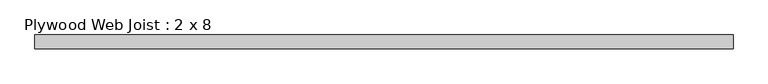
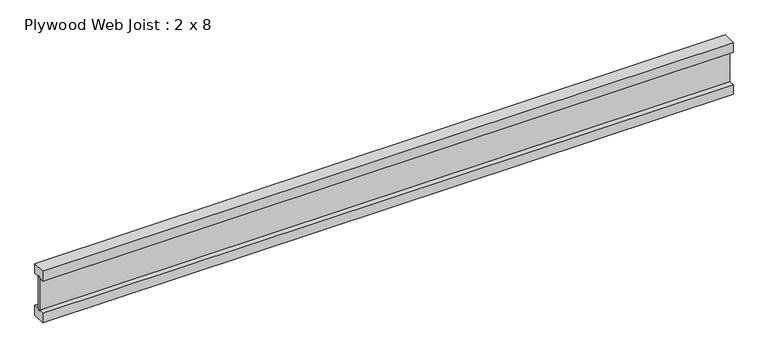
"""IFC4 building model written with IfcOpenShell, lengths in millimetres: beam geometry, Plywood Web Joist : 2 x 8."""

from ifc_helpers import new_model, si_unit, frame, origin, place, context, project, spatial, polyline, outline, extrude, source, transform, mapped, element, save


def plywood_web_joist_2_x_8_e6685f11(model_context):
    return source(origin(), model_context, "Body", "SweptSolid", [
        extrude(outline(polyline([(-25.4, 101.6), (25.4, 101.6), (25.4, 63.5), (4.7625, 63.5), (4.7625, 69.85), (-4.7625, 69.85), (-4.7625, 63.5), (-25.4, 63.5), (-25.4, 101.6)])), frame((-1284.2875, 0.0, 0.0), z_axis=(1.0, 0.0, 0.0), x_axis=(0.0, 1.0, 0.0)), (0.0, 0.0, 1.0), 2568.575),
        extrude(outline(polyline([(25.4, -63.5), (25.4, -101.6), (-25.4, -101.6), (-25.4, -63.5), (-4.7625, -63.5), (-4.7625, -69.1160374), (4.7625, -69.1160374), (4.7625, -63.5), (25.4, -63.5)])), frame((-1284.2875, 0.0, 0.0), z_axis=(1.0, 0.0, 0.0), x_axis=(0.0, 1.0, 0.0)), (0.0, 0.0, 1.0), 2568.575),
        extrude(outline(polyline([(1284.2875, 4.7625), (1284.2875, -4.7625), (-1284.2875, -4.7625), (-1284.2875, 4.7625), (1284.2875, 4.7625)])), frame((0.0, 0.0, -69.1160374), z_axis=(0.0, 0.0, 1.0), x_axis=(1.0, 0.0, 0.0)), (0.0, 0.0, 1.0), 138.9660374),
    ])


if __name__ == "__main__":
    model = new_model("IFC4")
    model_context = context("Model", 3, world=origin())
    ifc_project = project(units=[si_unit("LENGTHUNIT", "METRE", prefix="MILLI")], contexts=[model_context])
    site = spatial("IfcSite", under=ifc_project)
    building = spatial("IfcBuilding", under=site)
    placement = place(None, origin())
    plywood_web_joist_2_x_8_shape = plywood_web_joist_2_x_8_e6685f11(model_context)
    element("IfcBeam", 1, ObjectType="Plywood Web Joist : 2 x 8", at=placement, inside=building, context=model_context, shape_type="MappedRepresentation", body=[
        mapped(plywood_web_joist_2_x_8_shape, transform((0.0, 0.0, 0.0), x_axis=(1.0, 0.0, 0.0), y_axis=(0.0, 1.0, 0.0), z_axis=(0.0, 0.0, 1.0))),
    ])
    save(model, "model.ifc")

# Revit data of these elements
# Type "Plywood Web Joist : 2 x 8"
#   Assembly Code = "B10"
#   Length [instance default] = 5' - 0"
#   b = 0' - 2"
#   d = 0' - 8"
#   Structural Material [instance default] = Softwood, Lumber
# Element 1 (IfcBeam, "Plywood Web Joist : 2 x 8")
#   Materials on its faces: "Softwood, Lumber"
# Materials
#   "Softwood, Lumber": class "Wood", colour RGB 144 113 62, transparency 0, Description = "Pinus Echinata", Cost = 0
